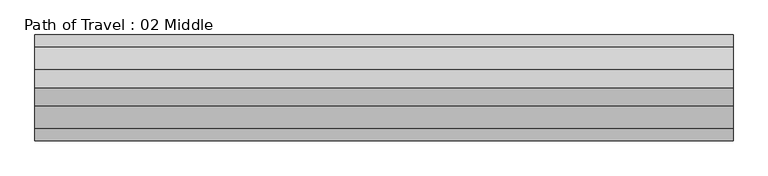
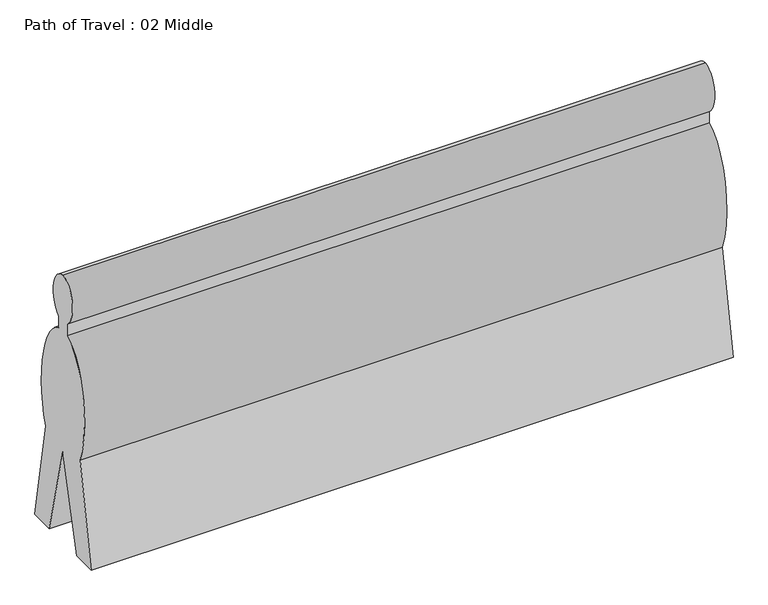
"""IFC4 building model written with IfcOpenShell, lengths in millimetres: proxy geometry, Path of Travel : 02 Middle."""

from ifc_helpers import new_model, si_unit, point, frame, origin, place, context, project, spatial, ellipse_curve, trimmed, source, transform, mapped, element, save
from ifc_brep_helpers import plane_surface, extruded_surface, advanced_brep


def path_of_travel_02_middle_3cefd49c(model_context):
    return source(origin(), model_context, "Body", "AdvancedBrep", [
        advanced_brep(
        [(227.5554837, 0.0, 1727.2), (227.5554837, 42.9018657, 1436.6534209), (227.5554837, 42.9018657, 1363.4763406), (227.5554837, 184.1186263, 643.4144547), (227.5554837, 297.5699544, 0.0), (227.5554837, 145.6574193, 0.0), (227.5554837, 0.0, 584.2), (227.5554837, -145.6574193, 0.0), (227.5554837, -297.5699544, 0.0), (227.5554837, -184.1186263, 643.4144547), (227.5554837, -42.9018657, 1363.4763406), (227.5554837, -42.9018657, 1436.6534209), (4159.8758778, 0.0, 1727.2), (4159.8758778, -42.9018657, 1436.6534209), (4159.8758778, -42.9018657, 1363.4763406), (4159.8758778, -184.1186263, 643.4144547), (4159.8758778, -297.5699544, 0.0), (4159.8758778, -145.6574193, 0.0), (4159.8758778, 0.0, 584.2), (4159.8758778, 145.6574193, 0.0), (4159.8758778, 297.5699544, 0.0), (4159.8758778, 184.1186263, 643.4144547), (4159.8758778, 42.9018657, 1363.4763406), (4159.8758778, 42.9018657, 1436.6534209)],
        [
            (0, 1, ellipse_curve(frame((227.5554837, 0.0, 1574.8), z_axis=(-1.0, 0.0, 0.0), x_axis=(0.0, 0.0, 1.0)), 152.4, 101.6)),
            (1, 2),
            (2, 3, ellipse_curve(frame((227.5554837, 0.0, 914.4), z_axis=(-1.0, 0.0, 0.0), x_axis=(0.0, 0.0, -1.0)), 457.2, 228.6)),
            (3, 4),
            (4, 5),
            (5, 6),
            (6, 7),
            (7, 8),
            (8, 9),
            (9, 10, ellipse_curve(frame((227.5554837, 0.0, 914.4), z_axis=(-1.0, 0.0, 0.0), x_axis=(0.0, 0.0, -1.0)), 457.2, 228.6)),
            (10, 11),
            (11, 0, ellipse_curve(frame((227.5554837, 0.0, 1574.8), z_axis=(-1.0, 0.0, 0.0), x_axis=(0.0, 0.0, 1.0)), 152.4, 101.6)),
            (12, 13, ellipse_curve(frame((4159.8758778, 0.0, 1574.8), z_axis=(1.0, 0.0, 0.0), x_axis=(0.0, 0.0, 1.0)), 152.4, 101.6)),
            (13, 14),
            (14, 15, ellipse_curve(frame((4159.8758778, 0.0, 914.4), z_axis=(1.0, 0.0, 0.0), x_axis=(0.0, 0.0, -1.0)), 457.2, 228.6)),
            (15, 16),
            (16, 17),
            (17, 18),
            (18, 19),
            (19, 20),
            (20, 21),
            (21, 22, ellipse_curve(frame((4159.8758778, 0.0, 914.4), z_axis=(1.0, 0.0, 0.0), x_axis=(0.0, 0.0, -1.0)), 457.2, 228.6)),
            (22, 23),
            (23, 12, ellipse_curve(frame((4159.8758778, 0.0, 1574.8), z_axis=(1.0, 0.0, 0.0), x_axis=(0.0, 0.0, 1.0)), 152.4, 101.6)),
            (0, 12),
            (23, 1),
            (22, 2),
            (21, 3),
            (20, 4),
            (19, 5),
            (18, 6),
            (17, 7),
            (16, 8),
            (15, 9),
            (14, 10),
            (13, 11),
        ],
        [
            plane_surface(frame((227.5554837, 0.0, 0.0), z_axis=(-1.0, 0.0, 0.0), x_axis=(0.0, 0.0, 1.0))),
            plane_surface(frame((4159.8758778, 0.0, 0.0), z_axis=(1.0, 0.0, 0.0), x_axis=(0.0, 0.0, 1.0))),
            extruded_surface(trimmed(ellipse_curve(frame((4159.8758778, 0.0, 1574.8), z_axis=(-1.0, 0.0, 0.0), x_axis=(0.0, 0.0, 1.0)), 152.4, 101.6), [point((4159.8758778, 0.0, 1727.2))], [point((4159.8758778, 42.9018657, 1436.6534209))], True, "CARTESIAN"), (-3932.3203941, 0.0, 0.0), 3932.3203941),
            plane_surface(frame((227.5554837, 42.9018657, 1436.6534209), z_axis=(0.0, 1.0, 0.0), x_axis=(1.0, 0.0, 0.0))),
            extruded_surface(trimmed(ellipse_curve(frame((4159.8758778, 0.0, 914.4), z_axis=(-1.0, 0.0, 0.0), x_axis=(0.0, 0.0, -1.0)), 457.2, 228.6), [point((4159.8758778, 42.9018657, 1363.4763406))], [point((4159.8758778, 184.1186263, 643.4144547))], True, "CARTESIAN"), (-3932.3203941, 0.0, 0.0), 3932.3203941),
            plane_surface(frame((227.5554837, 184.1186263, 643.4144547), z_axis=(0.0, 0.9848077530122078, 0.17364817766693205), x_axis=(1.0, 0.0, 0.0))),
            plane_surface(frame((227.5554837, 297.5699544, 0.0), z_axis=(0.0, 0.0, -1.0), x_axis=(1.0, 0.0, 0.0))),
            plane_surface(frame((227.5554837, 145.6574193, 0.0), z_axis=(0.0, -0.9702957262760199, -0.2419218955995739), x_axis=(1.0, 0.0, 0.0))),
            plane_surface(frame((227.5554837, 0.0, 584.2), z_axis=(0.0, 0.9702957262759961, -0.24192189559966923), x_axis=(1.0, 0.0, 0.0))),
            plane_surface(frame((227.5554837, -145.6574193, 0.0), z_axis=(0.0, 0.0, -1.0), x_axis=(1.0, 0.0, 0.0))),
            plane_surface(frame((227.5554837, -297.5699544, 0.0), z_axis=(0.0, -0.984807753012208, 0.17364817766693066), x_axis=(1.0, 0.0, 0.0))),
            extruded_surface(trimmed(ellipse_curve(frame((4159.8758778, 0.0, 914.4), z_axis=(-1.0, 0.0, 0.0), x_axis=(0.0, 0.0, -1.0)), 457.2, 228.6), [point((4159.8758778, -184.1186263, 643.4144547))], [point((4159.8758778, -42.9018657, 1363.4763406))], True, "CARTESIAN"), (-3932.3203941, 0.0, 0.0), 3932.3203941),
            plane_surface(frame((227.5554837, -42.9018657, 1363.4763406), z_axis=(0.0, -1.0, 0.0), x_axis=(1.0, 0.0, 0.0))),
            extruded_surface(trimmed(ellipse_curve(frame((4159.8758778, 0.0, 1574.8), z_axis=(-1.0, 0.0, 0.0), x_axis=(0.0, 0.0, 1.0)), 152.4, 101.6), [point((4159.8758778, -42.9018657, 1436.6534209))], [point((4159.8758778, 0.0, 1727.2))], True, "CARTESIAN"), (-3932.3203941, 0.0, 0.0), 3932.3203941),
        ],
        [
            (0, [[1, 2, 3, 4, 5, 6, 7, 8, 9, 10, 11, 12]]),
            (1, [[13, 14, 15, 16, 17, 18, 19, 20, 21, 22, 23, 24]]),
            (2, [[-1, 25, -24, 26]]),
            (3, [[-2, -26, -23, 27]]),
            (4, [[-3, -27, -22, 28]]),
            (5, [[-4, -28, -21, 29]]),
            (6, [[-5, -29, -20, 30]]),
            (7, [[-6, -30, -19, 31]]),
            (8, [[-7, -31, -18, 32]]),
            (9, [[-8, -32, -17, 33]]),
            (10, [[-9, -33, -16, 34]]),
            (11, [[-10, -34, -15, 35]]),
            (12, [[-11, -35, -14, 36]]),
            (13, [[-12, -36, -13, -25]]),
        ],
    ),
    ])


if __name__ == "__main__":
    model = new_model("IFC4")
    model_context = context("Model", 3, world=origin())
    ifc_project = project(units=[si_unit("LENGTHUNIT", "METRE", prefix="MILLI")], contexts=[model_context])
    site = spatial("IfcSite", under=ifc_project)
    building = spatial("IfcBuilding", under=site)
    placement = place(None, origin())
    path_of_travel_02_middle_shape = path_of_travel_02_middle_3cefd49c(model_context)
    element("IfcBuildingElementProxy", 1, Name="Path of Travel : 02 Middle", ObjectType="Path of Travel : 02 Middle", at=placement, inside=building, context=model_context, shape_type="MappedRepresentation", body=[
        mapped(path_of_travel_02_middle_shape, transform((0.0, 0.0, 0.0), x_axis=(1.0, 0.0, 0.0), y_axis=(0.0, 1.0, 0.0), z_axis=(0.0, 0.0, 1.0))),
    ])
    save(model, "model.ifc")

# Revit data of these elements
# Type "Path of Travel : 02 Middle"
#   Path of Egress [instance default] = 4' - 0"
#   built-in parameter 1001306 [instance default] = 4 (stored number, unit not read)
#   Dot at Start = no
#   Arrow in Middle = yes
#   Arrow at End = no
#   Egress Path = none
# Element 1 (IfcBuildingElementProxy, "Path of Travel : 02 Middle")
#   Path of Egress = 12' - 10.81576"
#   built-in parameter 1001306 = 12.9013 (stored number, unit not read)
#   Materials on its faces: "Egress Path Solid"
# Materials
#   "Egress Path Solid": class "Unassigned", colour RGB 255 128 64, transparency 0.75, Comments = "Rendering appearance not upgraded "
